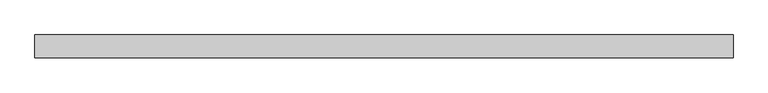
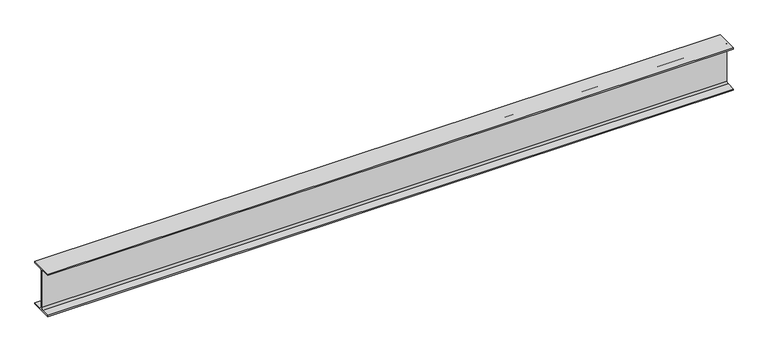
"""IFC4 building model written with IfcOpenShell, lengths in millimetres: beam geometry, 0912_Steel Framing_H-KSD3502 : H_SB_AR_S02_H-300x150x6.5x9_Stair."""

from ifc_helpers import new_model, si_unit, point, frame, frame_2d, origin, place, context, project, spatial, polyline, circle_curve, trimmed, segment, composite_curve, outline, extrude, source, transform, mapped, element, save


def beam_c94bab30(model_context):
    return source(origin(), model_context, "Body", "SweptSolid", [
        extrude(outline(composite_curve([segment(polyline([(75.0, -141.0), (75.0, -150.0), (-75.0, -150.0), (-75.0, -141.0), (-16.25, -141.0)]), True, "CONTINUOUS"), segment(trimmed(circle_curve(frame_2d((-16.25, -128.0)), 13.0), [point((-16.25, -141.0))], [point((-3.25, -128.0))], True, "CARTESIAN"), True, "CONTINUOUS"), segment(polyline([(-3.25, -128.0), (-3.25, 128.0)]), True, "CONTINUOUS"), segment(trimmed(circle_curve(frame_2d((-16.25, 128.0)), 13.0), [point((-3.25, 128.0))], [point((-16.25, 141.0))], True, "CARTESIAN"), True, "CONTINUOUS"), segment(polyline([(-16.25, 141.0), (-75.0, 141.0), (-75.0, 150.0), (75.0, 150.0), (75.0, 141.0), (16.25, 141.0)]), True, "CONTINUOUS"), segment(trimmed(circle_curve(frame_2d((16.25, 128.0)), 13.0), [point((16.25, 141.0))], [point((3.25, 128.0))], True, "CARTESIAN"), True, "CONTINUOUS"), segment(polyline([(3.25, 128.0), (3.25, -128.0)]), True, "CONTINUOUS"), segment(trimmed(circle_curve(frame_2d((16.25, -128.0)), 13.0), [point((3.25, -128.0))], [point((16.25, -141.0))], True, "CARTESIAN"), True, "CONTINUOUS"), segment(polyline([(16.25, -141.0), (75.0, -141.0)]), True, "CONTINUOUS")], self_intersect=False)), frame((-2306.6602947, 0.0, 0.0), z_axis=(1.0, 0.0, 0.0), x_axis=(0.0, 1.0, 0.0)), (0.0, 0.0, 1.0), 4574.4611041),
    ])


if __name__ == "__main__":
    model = new_model("IFC4")
    model_context = context("Model", 3, world=origin())
    ifc_project = project(units=[si_unit("LENGTHUNIT", "METRE", prefix="MILLI")], contexts=[model_context])
    site = spatial("IfcSite", under=ifc_project)
    building = spatial("IfcBuilding", under=site)
    placement = place(None, origin())
    beam_shape = beam_c94bab30(model_context)
    element("IfcBeam", 1, ObjectType="0912_Steel Framing_H-KSD3502 : H_SB_AR_S02_H-300x150x6.5x9_Stair", at=placement, inside=building, context=model_context, shape_type="MappedRepresentation", body=[
        mapped(beam_shape, transform((0.0, 0.0, 0.0), x_axis=(1.0, 0.0, 0.0), y_axis=(0.0, 1.0, 0.0), z_axis=(0.0, 0.0, 1.0))),
    ])
    save(model, "model.ifc")

# Revit data of these elements
# Type "0912_Steel Framing_H-KSD3502 : H_SB_AR_S02_H-300x150x6.5x9_Stair"
#   H_Q'ty Cal Type Tag = "SB-Q2"
#   H_WM Code_1 = "S01AA073-00001 |  | TON | Main Steel Structure Fabrication Work | Shelter/Building | Medium Steel - Standard |  |  |  |  |  |  | Material: (   ) | (90)KG/M>Weight≥(30)KG/M | S01AA073-00001 Main Steel Structure Fabrication Work Shelter/Building Medium Steel - Standard         | - Material: ( ASTM A36 )\n- (90)KG/M>Weight≥(30)KG/M"
#   H_WM Code_2 = "S03AA083-00001 |  | TON | Main Steel Structure Erection Work | Shelter/Building | Medium Steel |  |  |  |  |  |  | Material: (   ) | S03AA083-00001 Main Steel Structure Erection Work Shelter/Building Medium Steel         | - Material: ( ASTM A36 )"
#   H_WM Code_3 = "S01AA009-00001 |  | TON | Main Steel Structure Fabrication Work | Shelter/Building | Plates - Gusset, Stiffener, ETC | Material: (   ) | S01AA009-00001 Main Steel Structure Fabrication Work Shelter/Building Plates - Gusset, Stiffener, ETC         |"
#   H_WM Code_4 = "S41AA051-00001 |  | M2 | Steel Structure Paint Work | Shelter/Building | for Non-Fireproofed Steel Surface |  |  |  |  |  |  | Material: (   ) | S41AA051-00001 Steel Structure Paint Work Shelter/Building for Non-Fireproofed Steel Surface         |"
#   Width = 15.0 cm
#   Web Thickness = 0.65 cm
#   Web Fillet = 1.3 cm
#   Warping Constant = 107000.0 cm⁶
#   W = 0
#   Torsional Moment of Inertia = 9.9539 cm⁴
#   Section Area = 46.78 cm²
#   Plastic Modulus weak axis = 105.0 cm³
#   Plastic Modulus strong axis = 542.0 cm³
#   Perimeter = 1.17 m²/m
#   Nominal Weight = 36.70 kgf/m
#   Moment of Inertia weak axis = 508.00 cm⁴
#   Moment of Inertia strong axis = 7210.00 cm⁴
#   Height = 30.0 cm
#   Flange Thickness = 0.9 cm
#   Elastic Modulus weak axis = 67.7 cm³
#   Elastic Modulus strong axis = 481.0 cm³
#   Centroid Vertical = 15.0 cm
#   Centroid Horizontal = 7.5 cm
#   Ix = 72100000
#   Length [instance default] = 1524 mm
#   Zx = 542000
#   b = 150 mm
#   h = 300 mm
#   r = 13 mm
#   s = 6.5 mm
#   t = 9 mm
#   A = 0.004678 m²
#   Structural Material [instance default] = Steel, 45-345
#   Assembly Code = ""
# Element 1 (IfcBeam, "0912_Steel Framing_H-KSD3502 : H_SB_AR_S02_H-300x150x6.5x9_Stair")
#   Materials on its faces: "Steel, 45-345"
# Materials
#   "Steel, 45-345": class "Metal", colour RGB 189 187 185, transparency 0, Description = "Steel 345 MPa", Cost = 0
